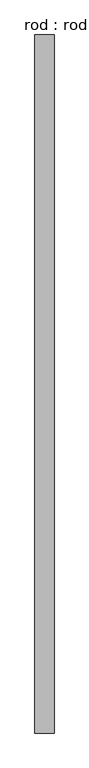
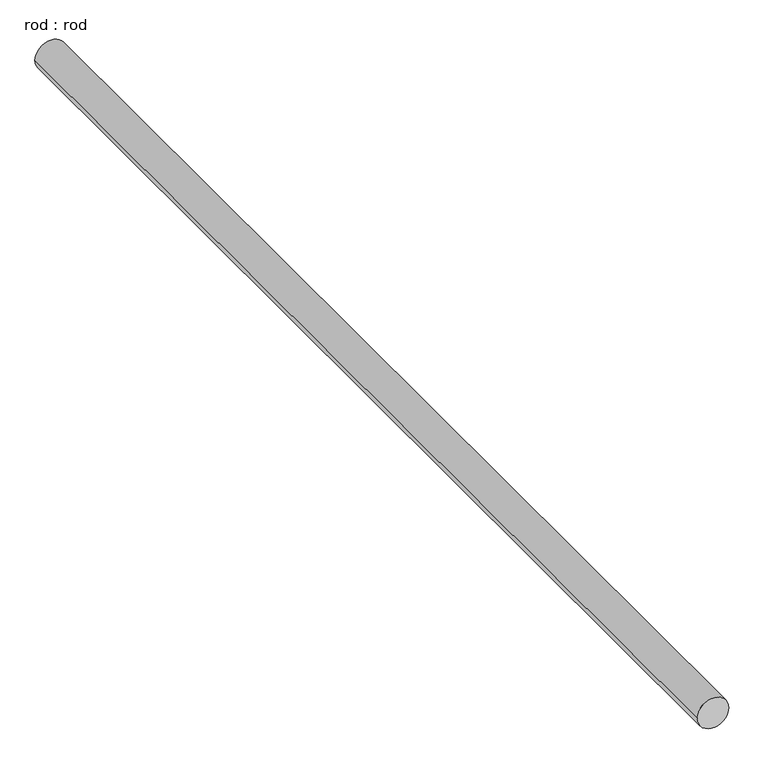
"""IFC4 building model written with IfcOpenShell, lengths in millimetres: proxy geometry, rod : rod."""

from ifc_helpers import new_model, si_unit, point, frame, frame_2d, origin, place, context, project, spatial, circle_curve, trimmed, segment, composite_curve, outline, extrude, source, transform, mapped, element, save


def rod_rod_f8087fb0(model_context):
    return source(origin(), model_context, "Body", "SweptSolid", [
        extrude(outline(composite_curve([segment(trimmed(circle_curve(frame_2d((0.0108462, 0.0)), 200.0), [point((0.0108462, 200.0))], [point((0.0108462, -200.0))], False, "CARTESIAN"), True, "CONTINUOUS"), segment(trimmed(circle_curve(frame_2d((0.0108462, 0.0)), 200.0), [point((0.0108462, -200.0))], [point((0.0108462, 200.0))], False, "CARTESIAN"), True, "CONTINUOUS")], self_intersect=False)), frame((0.0, -3190.115783, 0.0), z_axis=(0.0, 1.0, 0.0), x_axis=(0.0, 0.0, 1.0)), (0.0, 0.0, 1.0), 14565.6887967),
    ])


if __name__ == "__main__":
    model = new_model("IFC4")
    model_context = context("Model", 3, world=origin())
    ifc_project = project(units=[si_unit("LENGTHUNIT", "METRE", prefix="MILLI")], contexts=[model_context])
    site = spatial("IfcSite", under=ifc_project)
    building = spatial("IfcBuilding", under=site)
    placement = place(None, origin())
    rod_rod_shape = rod_rod_f8087fb0(model_context)
    element("IfcBuildingElementProxy", 1, Name="rod : rod", ObjectType="rod : rod", at=placement, inside=building, context=model_context, shape_type="MappedRepresentation", body=[
        mapped(rod_rod_shape, transform((0.0, 0.0, 0.0), x_axis=(1.0, 0.0, 0.0), y_axis=(0.0, 1.0, 0.0), z_axis=(0.0, 0.0, 1.0))),
    ])
    save(model, "model.ifc")

# Revit data of these elements
# Type "rod : rod"
#   Default Elevation = 0
